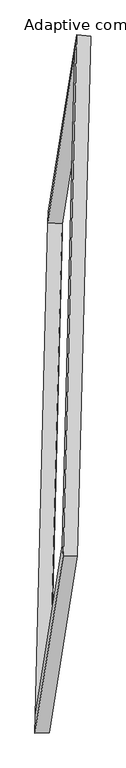
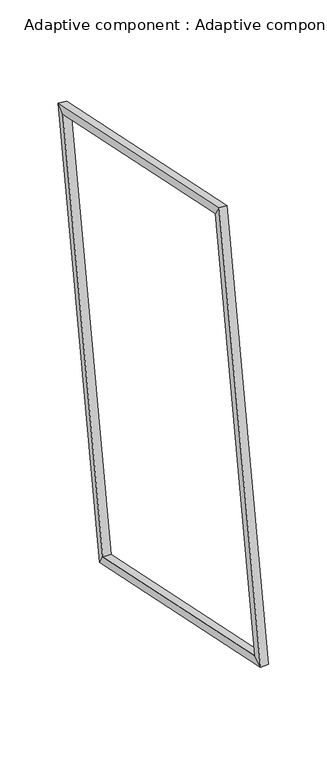
"""IFC4 building model written with IfcOpenShell, lengths in millimetres: proxy geometry, Adaptive component : Adaptive component."""

from ifc_helpers import new_model, si_unit, origin, place, context, project, spatial, faceted_brep, source, transform, mapped, element, save


def adaptive_component_adaptive_component_fc09e365(model_context):
    return source(origin(), model_context, "Body", "Brep", [
        faceted_brep([(67.305449, 1088.5213205, 2721.3362556), (131.9653956, 1082.5446098, 2717.0227902), (74.3662017, -1152.7276449, 3246.4500057), (9.5458616, -1152.9753844, 3252.2377404), (74.5058795, 1166.4645816, 2769.4274825), (13.4915701, -1201.3392718, 3330.2449839), (139.1658261, 1160.4878709, 2765.1140171), (78.3119102, -1201.0915323, 3324.4572492), (-48.8986333, -1925.1628087, -28.2264645), (-113.9532405, -1926.8785755, -28.6623132), (-114.761303, -2005.0318171, -76.94463), (-49.7066958, -2003.3160502, -76.5087813), (8.7005606, 310.1094461, -557.6536799), (-56.1936531, 314.6181294, -559.563798), (-53.7469935, 362.7720363, -637.7621315), (11.1472201, 358.263353, -635.8520134)], [[[0, 1, 2, 3]], [[4, 0, 3, 5]], [[6, 4, 5, 7]], [[1, 6, 7, 2]], [[3, 2, 8, 9]], [[5, 3, 9, 10]], [[7, 5, 10, 11]], [[2, 7, 11, 8]], [[9, 8, 12, 13]], [[10, 9, 13, 14]], [[11, 10, 14, 15]], [[8, 11, 15, 12]], [[13, 12, 1, 0]], [[14, 13, 0, 4]], [[15, 14, 4, 6]], [[12, 15, 6, 1]]]),
    ])


if __name__ == "__main__":
    model = new_model("IFC4")
    model_context = context("Model", 3, world=origin())
    ifc_project = project(units=[si_unit("LENGTHUNIT", "METRE", prefix="MILLI")], contexts=[model_context])
    site = spatial("IfcSite", under=ifc_project)
    building = spatial("IfcBuilding", under=site)
    placement = place(None, origin())
    adaptive_component_adaptive_component_shape = adaptive_component_adaptive_component_fc09e365(model_context)
    element("IfcBuildingElementProxy", 1, Name="Adaptive component : Adaptive component", ObjectType="Adaptive component : Adaptive component", at=placement, inside=building, context=model_context, shape_type="MappedRepresentation", body=[
        mapped(adaptive_component_adaptive_component_shape, transform((0.0, 0.0, 0.0), x_axis=(1.0, 0.0, 0.0), y_axis=(0.0, 1.0, 0.0), z_axis=(0.0, 0.0, 1.0))),
    ])
    save(model, "model.ifc")

# Revit data of these elements
# Type "Adaptive component : Adaptive component"
#   r [instance default] = 2063.125 mm
#   2r [instance default] = 4126.251 mm
#   Number [instance default] = 5
#   Default Elevation = 0
# Element 1 (IfcBuildingElementProxy, "Adaptive component : Adaptive component")
#   r = 2130.723 mm
#   2r = 4261.447 mm
#   Number = 7
